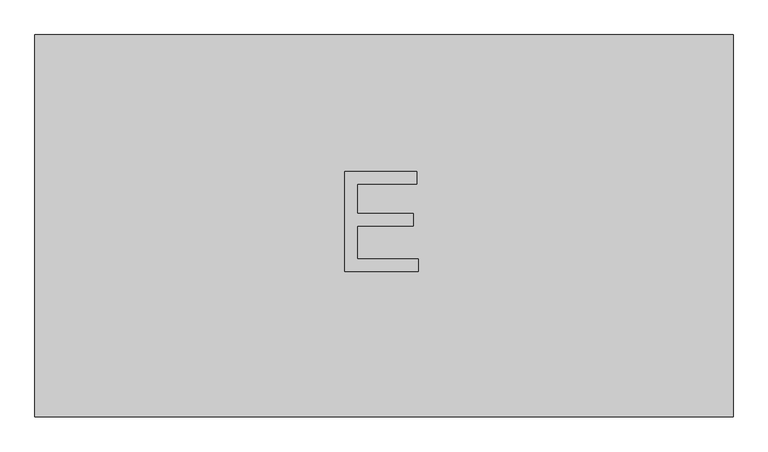
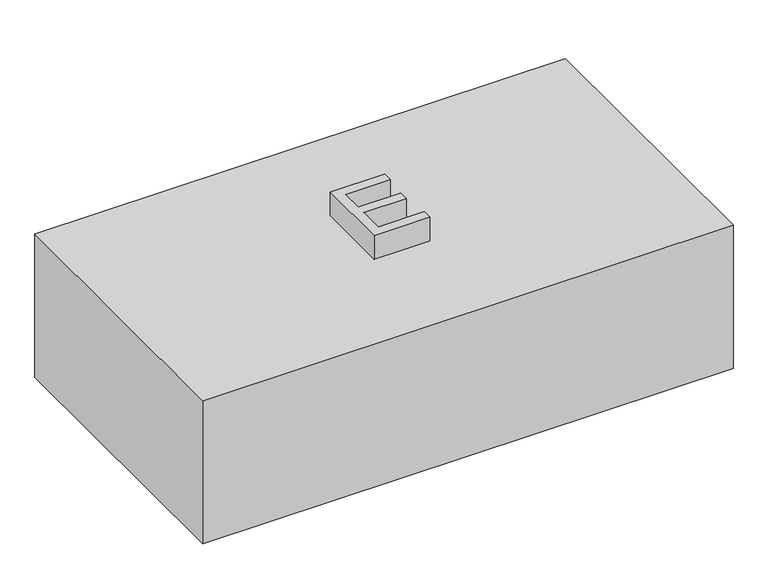
"""IFC4 building model written with IfcOpenShell, lengths in millimetres: proxy geometry, The Messy Family E : The Messy Family E."""

from ifc_helpers import new_model, si_unit, frame, origin, origin_with_axes, place, context, project, spatial, polyline, outline, extrude, source, transform, mapped, element, save


def generic_models_e1a2475d(model_context):
    return source(origin(), model_context, "Body", "SweptSolid", [
        extrude(outline(polyline([(541.9415527, 284.565081), (541.9415527, -299.634919), (-524.8584473, -299.634919), (-524.8584473, 284.565081), (541.9415527, 284.565081)])), origin_with_axes(), (0.0, 0.0, 1.0), 304.8),
        extrude(outline(polyline([(-51.7602961, -77.2556777), (-51.7602961, 75.839739), (58.2770347, 75.839739), (58.2770347, 56.7028119), (-32.623369, 56.7028119), (-32.623369, 11.2526101), (53.4928029, 11.2526101), (53.4928029, -7.884317), (-32.623369, -7.884317), (-32.623369, -58.1187506), (60.6691506, -58.1187506), (60.6691506, -77.2556777), (-51.7602961, -77.2556777)])), frame((0.0, 0.0, 304.8), z_axis=(0.0, 0.0, 1.0), x_axis=(1.0, 0.0, 0.0)), (0.0, 0.0, 1.0), 50.8),
    ])


if __name__ == "__main__":
    model = new_model("IFC4")
    model_context = context("Model", 3, world=origin())
    ifc_project = project(units=[si_unit("LENGTHUNIT", "METRE", prefix="MILLI")], contexts=[model_context])
    site = spatial("IfcSite", under=ifc_project)
    building = spatial("IfcBuilding", under=site)
    placement = place(None, origin())
    generic_models_shape = generic_models_e1a2475d(model_context)
    element("IfcBuildingElementProxy", 1, Name="The Messy Family E : The Messy Family E", ObjectType="The Messy Family E : The Messy Family E", at=placement, inside=building, context=model_context, shape_type="MappedRepresentation", body=[
        mapped(generic_models_shape, transform((0.0, 0.0, 0.0), x_axis=(1.0, 0.0, 0.0), y_axis=(0.0, 1.0, 0.0), z_axis=(0.0, 0.0, 1.0))),
    ])
    save(model, "model.ifc")

# Revit data of these elements
# Type "The Messy Family E : The Messy Family E"
#   TBC-Parameter 2 = ""
#   TBC-Parameter 1 = ""
#   Other Company Parameter 2 = ""
#   Other Company Parameter 1 = ""
#   TBC-Parameter 3 = 2' - 0"
#   Other Company Parameter 3 = 1' - 0"
#   Default Elevation = 0
